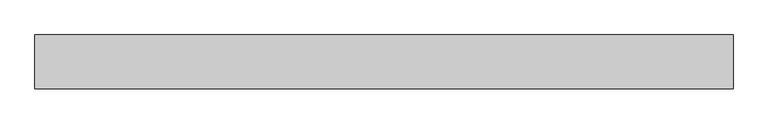
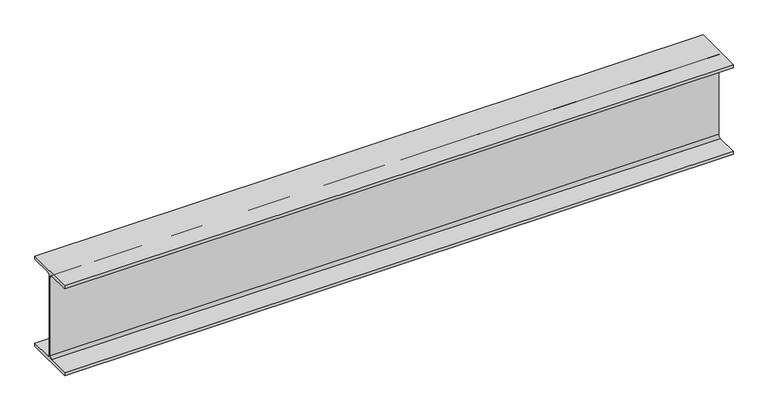
"""IFC4 building model written with IfcOpenShell, lengths in millimetres: beam geometry, Old_Steel Beam_H-KSD3502 : H_SB_ASB_H-194×150x6x9."""

import ifcopenshell
import ifcopenshell.guid

model = None  # the IFC model being written
_history = None  # IfcOwnerHistory: only IFC2X3 demands one
_inside = {}  # id of a spatial element -> (the spatial element, [elements in it])
_under = {}  # id of a project, library or spatial element -> (it, [spatial elements below it])
_declared = {}  # id of a project -> (the project, [libraries it declares])
_typed = {}  # id of a type object -> (the type object, [elements of that type])
_made_of = {}  # id of a material, layer set ... -> (it, [elements and type objects made of it])


def new_model(schema):
    """Start an empty IFC model of exactly this schema.

    Asked for "IFC4X3", IfcOpenShell would pick the latest addendum, in which some entities
    have other attributes; the version numbers below select the first issue.
    IFC2X3 requires an IfcOwnerHistory on every rooted entity: one is made here for all.
    """
    global model, _history
    if schema == "IFC4X3":
        model = ifcopenshell.file(schema_version=(4, 3, 0, 0))
    else:
        model = ifcopenshell.file(schema=schema)
    _inside.clear()
    _under.clear()
    _declared.clear()
    _typed.clear()
    _made_of.clear()
    _history = None
    if model.schema == "IFC2X3":
        org = make("IfcOrganization", Name="unknown")
        user = make(
            "IfcPersonAndOrganization",
            ThePerson=make("IfcPerson", FamilyName="unknown"),
            TheOrganization=org,
        )
        app = make(
            "IfcApplication",
            ApplicationDeveloper=org,
            Version="unknown",
            ApplicationFullName="unknown",
            ApplicationIdentifier="unknown",
        )
        _history = make(
            "IfcOwnerHistory",
            OwningUser=user,
            OwningApplication=app,
            ChangeAction="ADDED",
            CreationDate=0,
        )
    return model


def make(cls, **values):
    """One entity of the class cls with the attributes given. An attribute that is None is left unset."""
    return model.create_entity(
        cls, **{name: value for name, value in values.items() if value is not None}
    )


def rooted(cls, **values):
    """An entity with a GlobalId (a new one), such as an element, a storey or a relation."""
    return make(cls, GlobalId=ifcopenshell.guid.new(), OwnerHistory=_history, **values)


def si_unit(unit_type, name, prefix=None):
    """IfcSIUnit, for example si_unit("LENGTHUNIT", "METRE", prefix="MILLI")."""
    return make("IfcSIUnit", UnitType=unit_type, Prefix=prefix, Name=name)


def assignment(units):
    """IfcUnitAssignment: the units of a project."""
    return None if units is None else make("IfcUnitAssignment", Units=units)


def point(xyz):
    """IfcCartesianPoint."""
    return None if xyz is None else make("IfcCartesianPoint", Coordinates=xyz)


def direction(xyz):
    """IfcDirection."""
    return None if xyz is None else make("IfcDirection", DirectionRatios=xyz)


def frame(location, z_axis=None, x_axis=None):
    """IfcAxis2Placement3D, a coordinate frame: its origin and axes. An axis left out is left unset."""
    return make(
        "IfcAxis2Placement3D",
        Location=point(location),
        Axis=direction(z_axis),
        RefDirection=direction(x_axis),
    )


def frame_2d(location, x_axis=None):
    """IfcAxis2Placement2D, a coordinate frame in the plane: its origin and x axis."""
    return make(
        "IfcAxis2Placement2D", Location=point(location), RefDirection=direction(x_axis)
    )


def origin():
    """The frame at (0, 0, 0) with its axes left unset."""
    return frame((0.0, 0.0, 0.0))


def place(relative_to, where):
    """IfcLocalPlacement: puts the frame where relative to a parent placement (None: the world)."""
    return make(
        "IfcLocalPlacement", PlacementRelTo=relative_to, RelativePlacement=where
    )


def context(
    kind, dimensions, precision=None, world=None, true_north=None, identifier=None
):
    """IfcGeometricRepresentationContext, for example the 3D "Model" context."""
    return make(
        "IfcGeometricRepresentationContext",
        ContextIdentifier=identifier,
        ContextType=kind,
        CoordinateSpaceDimension=dimensions,
        Precision=precision,
        WorldCoordinateSystem=world,
        TrueNorth=true_north,
    )


def project(units=None, contexts=None):
    """IfcProject with its units and contexts."""
    return rooted(
        "IfcProject",
        Name="project",
        RepresentationContexts=contexts,
        UnitsInContext=assignment(units),
    )


def spatial(cls, under=None, at=None, **own):
    """A site, building, storey or space (cls), placed at a placement, below another one or the project."""
    s = rooted(cls, ObjectPlacement=at, **own)
    if under is not None:
        _under.setdefault(under.id(), (under, []))[1].append(s)
    return s


def polyline(points):
    """IfcPolyline through the points."""
    return make("IfcPolyline", Points=[point(p) for p in points])


def circle_curve(where, radius):
    """IfcCircle in the frame where."""
    return make("IfcCircle", Position=where, Radius=radius)


def trimmed(basis, trim1, trim2, sense, master):
    """IfcTrimmedCurve: the piece of a basis curve between two trims."""
    return make(
        "IfcTrimmedCurve",
        BasisCurve=basis,
        Trim1=trim1,
        Trim2=trim2,
        SenseAgreement=sense,
        MasterRepresentation=master,
    )


def segment(curve, same_sense, transition):
    """IfcCompositeCurveSegment."""
    return make(
        "IfcCompositeCurveSegment",
        Transition=transition,
        SameSense=same_sense,
        ParentCurve=curve,
    )


def composite_curve(segments, self_intersect=None):
    """IfcCompositeCurve: segments joined end to end."""
    return make("IfcCompositeCurve", Segments=segments, SelfIntersect=self_intersect)


def outline(outer, holes=None, kind="AREA"):
    """IfcArbitraryClosedProfileDef: a profile drawn as a closed curve; with holes, ...WithVoids."""
    if holes is None:
        return make("IfcArbitraryClosedProfileDef", ProfileType=kind, OuterCurve=outer)
    return make(
        "IfcArbitraryProfileDefWithVoids",
        ProfileType=kind,
        OuterCurve=outer,
        InnerCurves=holes,
    )


def extrude(swept, where, along, depth):
    """IfcExtrudedAreaSolid: the profile swept, set in the frame where, extruded along a direction by depth."""
    return make(
        "IfcExtrudedAreaSolid",
        SweptArea=swept,
        Position=where,
        ExtrudedDirection=direction(along),
        Depth=depth,
    )


def shape(context_of_items, identifier, shape_type, items):
    """IfcShapeRepresentation: the items that make up one representation, for example the "Body"."""
    return make(
        "IfcShapeRepresentation",
        ContextOfItems=context_of_items,
        RepresentationIdentifier=identifier,
        RepresentationType=shape_type,
        Items=items,
    )


def source(mapping_origin, context_of_items, identifier, shape_type, items):
    """IfcRepresentationMap: a shape defined once, which mapped items show again and again."""
    return make(
        "IfcRepresentationMap",
        MappingOrigin=mapping_origin,
        MappedRepresentation=shape(context_of_items, identifier, shape_type, items),
    )


def transform(
    local_origin,
    x_axis=None,
    y_axis=None,
    z_axis=None,
    scale=None,
    scale2=None,
    scale3=None,
    uniform=True,
):
    """IfcCartesianTransformationOperator3D, or its non-uniform kind. x_axis, y_axis, z_axis: its Axis1, 2, 3."""
    if uniform:
        return make(
            "IfcCartesianTransformationOperator3D",
            Axis1=direction(x_axis),
            Axis2=direction(y_axis),
            LocalOrigin=point(local_origin),
            Scale=scale,
            Axis3=direction(z_axis),
        )
    return make(
        "IfcCartesianTransformationOperator3DnonUniform",
        Axis1=direction(x_axis),
        Axis2=direction(y_axis),
        LocalOrigin=point(local_origin),
        Scale=scale,
        Axis3=direction(z_axis),
        Scale2=scale2,
        Scale3=scale3,
    )


def mapped(mapping_source, mapping_target):
    """IfcMappedItem: shows the shape of a source again, moved by a transform."""
    return make(
        "IfcMappedItem", MappingSource=mapping_source, MappingTarget=mapping_target
    )


def made_of(thing, what):
    """Note that an element or type object is made of a material, layer set ...; save() writes the relation."""
    if what is not None:
        _made_of.setdefault(what.id(), (what, []))[1].append(thing)
    return thing


def element(
    cls,
    number,
    at=None,
    inside=None,
    cuts=None,
    type_object=None,
    material=None,
    context=None,
    identifier="Body",
    shape_type=None,
    held_by="IfcProductDefinitionShape",
    body=None,
    shapes=None,
    **own,
):
    """One element of the class cls, such as IfcWall. Its Tag is "e" and its number.

    at: its placement. inside: the storey or other place that contains it. cuts: it is an
    opening in that element (IfcRelVoidsElement). A single representation is given by context,
    identifier, shape_type and body (its items); several are given by shapes. held_by: the class
    of the entity that holds the representations. save() writes the other relations.
    """
    e = rooted(cls, Tag="e%d" % number, ObjectPlacement=at, **own)
    if body is not None:
        shapes = [shape(context, identifier, shape_type, body)]
    if shapes is not None:
        e.Representation = make(held_by, Representations=shapes)
    if inside is not None:
        _inside.setdefault(inside.id(), (inside, []))[1].append(e)
    if cuts is not None:
        rooted(
            "IfcRelVoidsElement", RelatingBuildingElement=cuts, RelatedOpeningElement=e
        )
    if type_object is not None:
        _typed.setdefault(type_object.id(), (type_object, []))[1].append(e)
    return made_of(e, material)


def aggregate(whole, parts):
    """IfcRelAggregates: a whole, such as a stair, and the parts it consists of."""
    return rooted("IfcRelAggregates", RelatingObject=whole, RelatedObjects=parts)


def save(model, path):
    """Write the relations noted so far, then the file.

    IfcRelAggregates (storeys below a building ...), IfcRelContainedInSpatialStructure (elements
    in a storey), IfcRelDefinesByType, IfcRelAssociatesMaterial and IfcRelDeclares: one each for
    every whole, place, type object, material and project.
    """
    for whole, parts in _under.values():
        aggregate(whole, parts)
    for where, things in _inside.values():
        rooted(
            "IfcRelContainedInSpatialStructure",
            RelatedElements=things,
            RelatingStructure=where,
        )
    for kind, things in _typed.values():
        rooted("IfcRelDefinesByType", RelatedObjects=things, RelatingType=kind)
    for what, things in _made_of.values():
        rooted("IfcRelAssociatesMaterial", RelatedObjects=things, RelatingMaterial=what)
    for by, libraries in _declared.values():
        rooted("IfcRelDeclares", RelatingContext=by, RelatedDefinitions=libraries)
    model.write(path)


def beam_825be00d(model_context):
    return source(origin(), model_context, "Body", "SweptSolid", [
        extrude(outline(composite_curve([segment(polyline([(-82.5, -141.5), (-11.9, -141.5)]), True, "CONTINUOUS"), segment(trimmed(circle_curve(frame_2d((-11.9, -132.6)), 8.9), [point((-11.9, -141.5))], [point((-3.0, -132.6))], True, "CARTESIAN"), True, "CONTINUOUS"), segment(polyline([(-3.0, -132.6), (-3.0, 132.6)]), True, "CONTINUOUS"), segment(trimmed(circle_curve(frame_2d((-11.9, 132.6)), 8.9), [point((-3.0, 132.6))], [point((-11.9, 141.5))], True, "CARTESIAN"), True, "CONTINUOUS"), segment(polyline([(-11.9, 141.5), (-82.5, 141.5), (-82.5, 151.7), (82.5, 151.7), (82.5, 141.5), (11.9, 141.5)]), True, "CONTINUOUS"), segment(trimmed(circle_curve(frame_2d((11.9, 132.6)), 8.9), [point((11.9, 141.5))], [point((3.0, 132.6))], True, "CARTESIAN"), True, "CONTINUOUS"), segment(polyline([(3.0, 132.6), (3.0, -132.6)]), True, "CONTINUOUS"), segment(trimmed(circle_curve(frame_2d((11.9, -132.6)), 8.9), [point((3.0, -132.6))], [point((11.9, -141.5))], True, "CARTESIAN"), True, "CONTINUOUS"), segment(polyline([(11.9, -141.5), (82.5, -141.5), (82.5, -151.7), (-82.5, -151.7), (-82.5, -141.5)]), True, "CONTINUOUS")], self_intersect=False)), frame((-1067.7446443, 0.0, 0.0), z_axis=(1.0, 0.0, 0.0), x_axis=(0.0, 1.0, 0.0)), (0.0, 0.0, 1.0), 2135.4892885),
    ])


if __name__ == "__main__":
    model = new_model("IFC4")
    model_context = context("Model", 3, world=origin())
    ifc_project = project(units=[si_unit("LENGTHUNIT", "METRE", prefix="MILLI")], contexts=[model_context])
    site = spatial("IfcSite", under=ifc_project)
    building = spatial("IfcBuilding", under=site)
    placement = place(None, origin())
    beam_shape = beam_825be00d(model_context)
    element("IfcBeam", 1, ObjectType="Old_Steel Beam_H-KSD3502 : H_SB_ASB_H-194×150x6x9", at=placement, inside=building, context=model_context, shape_type="MappedRepresentation", body=[
        mapped(beam_shape, transform((0.0, 0.0, 0.0), x_axis=(1.0, 0.0, 0.0), y_axis=(0.0, 1.0, 0.0), z_axis=(0.0, 0.0, 1.0))),
    ])
    save(model, "model.ifc")

# Revit data of these elements
# Type "Old_Steel Beam_H-KSD3502 : H_SB_ASB_H-194×150x6x9"
#   Width = 15.0 cm
#   Web Thickness = 0.6 cm
#   Web Fillet = 1.3 cm
#   Warping Constant = 43316.0 cm⁶
#   Torsional Moment of Inertia = 8.622 cm⁴
#   Torsional Modulus = 1.0 cm³
#   Section Area = 39.01 cm²
#   Plastic Modulus weak axis = 104.0 cm³
#   Plastic Modulus strong axis = 309.0 cm³
#   Perimeter = 0.95 m²/m
#   Nominal Weight = 30.60 kgf/m
#   Moment of Inertia weak axis = 507.00 cm⁴
#   Moment of Inertia strong axis = 2690.00 cm⁴
#   Height = 19.4 cm
#   Flange Thickness = 0.9 cm
#   Elastic Modulus weak axis = 67.6 cm³
#   Elastic Modulus strong axis = 277.0 cm³
#   Centroid Vertical = 9.7 cm
#   Centroid Horizontal = 7.5 cm
#   Length [instance default] = 1.5240 m
#   Structural Material [instance default] = Steel, 45-345
#   Assembly Code = ""
# Element 1 (IfcBeam, "Old_Steel Beam_H-KSD3502 : H_SB_ASB_H-194×150x6x9")
#   Structural Material = none
# Materials
#   "Steel, 45-345": class "Metal", colour RGB 189 187 185, transparency 0, Description = "Steel 345 MPa", Cost = 0
